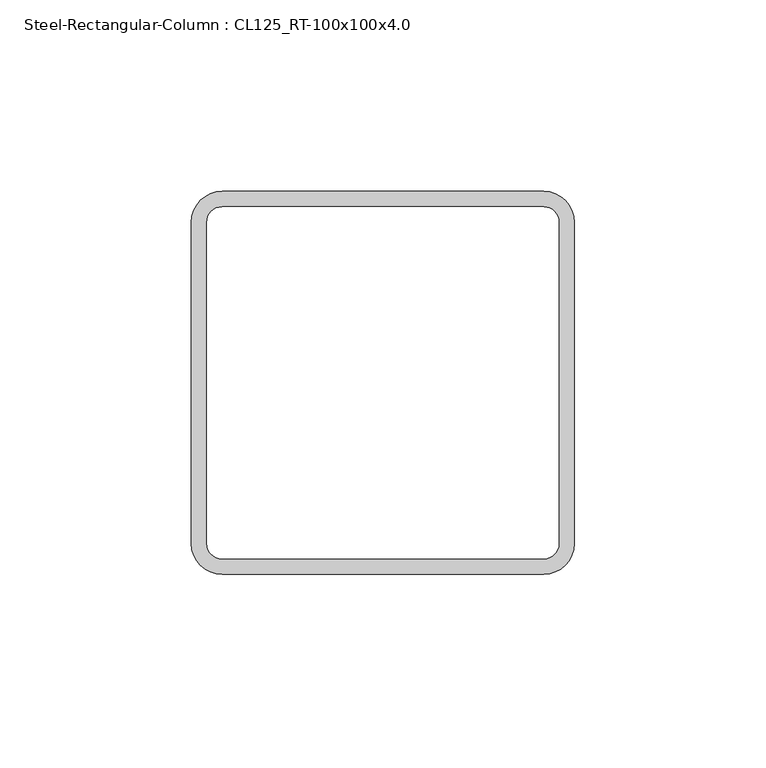
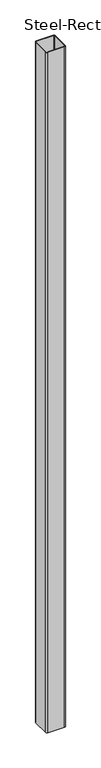
"""IFC4 building model written with IfcOpenShell, lengths in millimetres: column geometry, Steel-Rectangular-Column : CL125_RT-100x100x4.0."""

from ifc_helpers import new_model, si_unit, point, frame, frame_2d, origin, place, context, project, spatial, polyline, circle_curve, trimmed, segment, composite_curve, outline, extrude, source, transform, mapped, element, save


def steel_rectangular_column_cl125_rt_100x100x4_0_aaa137b4(model_context):
    return source(origin(), model_context, "Body", "SweptSolid", [
        extrude(outline(composite_curve([segment(trimmed(circle_curve(frame_2d((42.0, 42.0)), 8.0), [point((42.0, 50.0))], [point((50.0, 42.0))], False, "CARTESIAN"), True, "CONTINUOUS"), segment(polyline([(50.0, 42.0), (50.0, -42.0)]), True, "CONTINUOUS"), segment(trimmed(circle_curve(frame_2d((42.0, -42.0)), 8.0), [point((50.0, -42.0))], [point((42.0, -50.0))], False, "CARTESIAN"), True, "CONTINUOUS"), segment(polyline([(42.0, -50.0), (-42.0, -50.0)]), True, "CONTINUOUS"), segment(trimmed(circle_curve(frame_2d((-42.0, -42.0)), 8.0), [point((-42.0, -50.0))], [point((-50.0, -42.0))], False, "CARTESIAN"), True, "CONTINUOUS"), segment(polyline([(-50.0, -42.0), (-50.0, 42.0)]), True, "CONTINUOUS"), segment(trimmed(circle_curve(frame_2d((-42.0, 42.0)), 8.0), [point((-50.0, 42.0))], [point((-42.0, 50.0))], False, "CARTESIAN"), True, "CONTINUOUS"), segment(polyline([(-42.0, 50.0), (42.0, 50.0)]), True, "CONTINUOUS")], self_intersect=False), holes=[composite_curve([segment(polyline([(42.0, 46.0), (-42.0, 46.0)]), True, "CONTINUOUS"), segment(trimmed(circle_curve(frame_2d((-42.0, 42.0)), 4.0), [point((-42.0, 46.0))], [point((-46.0, 42.0))], True, "CARTESIAN"), True, "CONTINUOUS"), segment(polyline([(-46.0, 42.0), (-46.0, -42.0)]), True, "CONTINUOUS"), segment(trimmed(circle_curve(frame_2d((-42.0, -42.0)), 4.0), [point((-46.0, -42.0))], [point((-42.0, -46.0))], True, "CARTESIAN"), True, "CONTINUOUS"), segment(polyline([(-42.0, -46.0), (42.0, -46.0)]), True, "CONTINUOUS"), segment(trimmed(circle_curve(frame_2d((42.0, -42.0)), 4.0), [point((42.0, -46.0))], [point((46.0, -42.0))], True, "CARTESIAN"), True, "CONTINUOUS"), segment(polyline([(46.0, -42.0), (46.0, 42.0)]), True, "CONTINUOUS"), segment(trimmed(circle_curve(frame_2d((42.0, 42.0)), 4.0), [point((46.0, 42.0))], [point((42.0, 46.0))], True, "CARTESIAN"), True, "CONTINUOUS")], self_intersect=False)]), frame((0.0, 0.0, 1400.0), z_axis=(0.0, 0.0, 1.0), x_axis=(1.0, 0.0, 0.0)), (0.0, 0.0, 1.0), 3600.0),
    ])


if __name__ == "__main__":
    model = new_model("IFC4")
    model_context = context("Model", 3, world=origin())
    ifc_project = project(units=[si_unit("LENGTHUNIT", "METRE", prefix="MILLI")], contexts=[model_context])
    site = spatial("IfcSite", under=ifc_project)
    building = spatial("IfcBuilding", under=site)
    placement = place(None, origin())
    steel_rectangular_column_cl125_rt_100x100x4_0_shape = steel_rectangular_column_cl125_rt_100x100x4_0_aaa137b4(model_context)
    element("IfcColumn", 1, ObjectType="Steel-Rectangular-Column : CL125_RT-100x100x4.0", at=placement, inside=building, context=model_context, shape_type="MappedRepresentation", body=[
        mapped(steel_rectangular_column_cl125_rt_100x100x4_0_shape, transform((0.0, 0.0, 0.0), x_axis=(1.0, 0.0, 0.0), y_axis=(0.0, 1.0, 0.0), z_axis=(0.0, 0.0, 1.0))),
    ])
    save(model, "model.ifc")

# Revit data of these elements
# Type "Steel-Rectangular-Column : CL125_RT-100x100x4.0"
#   Surface Area = 0.386 m²/m
#   b = 100 mm
#   h = 100 mm
#   tr = 8 mm
#   t = 4 mm
#   Section Area = 14.95 cm²
#   Mass per Unit Length = 11.70 kg/m
#   hec_material4 [instance default] = none
#   hec_material3 [instance default] = none
#   hec_material2 [instance default] = none
#   hec_material1 [instance default] = none
#   Structural Material [instance default] = Steel, 45-345
# Element 1 (IfcColumn, "Steel-Rectangular-Column : CL125_RT-100x100x4.0")
#   Structural Material = S01AA007-00001_Main Steel Structure Fabrication Work_Shelter/Building_Girth & Purlin
#   Materials on its faces: "S01AA007-00001_Main Steel Structure Fabrication Work_Shelter/Building_Girth & Purlin"
# Materials
#   "Steel, 45-345": class "Metal", colour RGB 189 187 185, transparency 0, Description = "Steel 345 MPa", Cost = 0
#   "S01AA007-00001_Main Steel Structure Fabrication Work_Shelter/Building_Girth & Purlin": class "Metal", colour RGB 120 120 120, transparency 0, Comments = "(30KG/M>Weight)", Description = "Structural steel 50ksi", W00) Work Master Code = "S01AA007-00001", W01) Work Master_Lv1 = "Main Steel Structure Fabrication Work", W02) Work Master_Lv2 = "Shelter/Building", W03) Work Master_Spec.1 = "Girth & Purlin", Cost = 0
